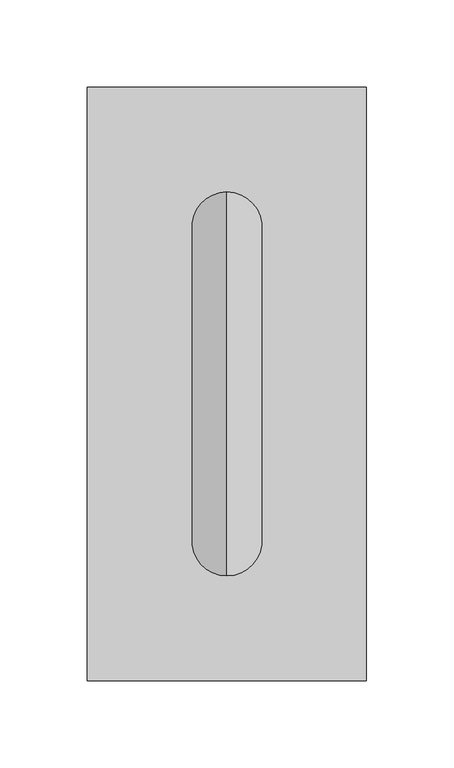
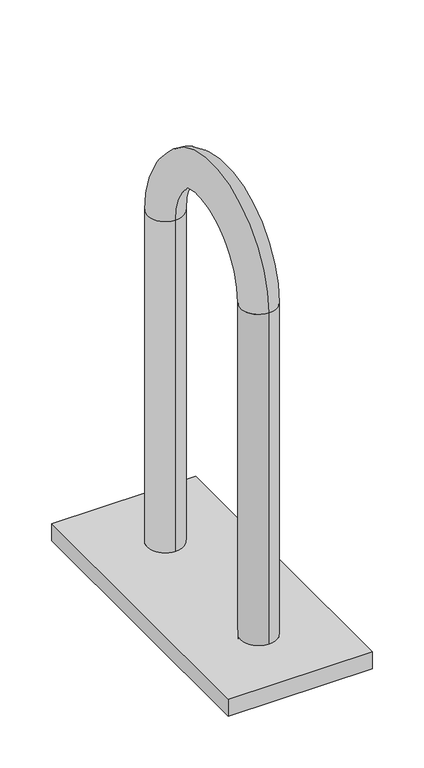
"""IFC4 building model written with IfcOpenShell, lengths in millimetres: proxy geometry, Опорный поручень : Опорный поручень для раковины."""

from ifc_helpers import new_model, si_unit, point, frame, origin, origin_with_axes, place, context, project, spatial, polyline, circle_curve, ellipse_curve, trimmed, outline, extrude, source, transform, mapped, element, save
from ifc_brep_helpers import plane_surface, cylinder_surface, revolved_surface, advanced_brep


def mechanical_equipment_83d53407(model_context):
    return source(origin(), model_context, "Body", "SolidModel", [
        extrude(outline(polyline([(80.0, 170.0), (80.0, -170.0), (-80.0, -170.0), (-80.0, 170.0), (80.0, 170.0)])), origin_with_axes(), (0.0, 0.0, 1.0), 20.0),
        advanced_brep(
        [(0.0, 110.0, 0.0), (0.0, 70.0, 0.0), (0.0, 110.0, 410.0), (0.0, 70.0, 410.0), (0.0, -70.0, 410.0), (0.0, -110.0, 410.0), (0.0, -110.0, 0.0), (0.0, -70.0, 0.0)],
        [
            (0, 1, circle_curve(frame((0.0, 90.0, 0.0), z_axis=(0.0, 0.0, -1.0), x_axis=(0.0, -1.0, 0.0)), 20.0)),
            (1, 0, circle_curve(frame((0.0, 90.0, 0.0), z_axis=(0.0, 0.0, -1.0), x_axis=(0.0, -1.0, 0.0)), 20.0)),
            (0, 2),
            (2, 3, circle_curve(frame((0.0, 90.0, 410.0), z_axis=(0.0, 0.0, -1.0), x_axis=(0.0, -1.0, 0.0)), 20.0)),
            (3, 1),
            (3, 2, circle_curve(frame((0.0, 90.0, 410.0), z_axis=(0.0, 0.0, -1.0), x_axis=(0.0, -1.0, 0.0)), 20.0)),
            (4, 3, circle_curve(frame((0.0, 0.0, 410.0), z_axis=(-1.0, 0.0, 0.0), x_axis=(0.0, 1.0, 0.0)), 70.0)),
            (2, 5, circle_curve(frame((0.0, 0.0, 410.0), z_axis=(1.0, 0.0, 0.0), x_axis=(0.0, 1.0, 0.0)), 110.0)),
            (5, 4, circle_curve(frame((0.0, -90.0, 410.0), z_axis=(0.0, 0.0, 1.0), x_axis=(0.0, 1.0, 0.0)), 20.0)),
            (4, 5, circle_curve(frame((0.0, -90.0, 410.0), z_axis=(0.0, 0.0, 1.0), x_axis=(0.0, 1.0, 0.0)), 20.0)),
            (6, 7, circle_curve(frame((0.0, -90.0, 0.0), z_axis=(0.0, 0.0, -1.0), x_axis=(0.0, 1.0, 0.0)), 20.0)),
            (7, 6, circle_curve(frame((0.0, -90.0, 0.0), z_axis=(0.0, 0.0, -1.0), x_axis=(0.0, 1.0, 0.0)), 20.0)),
            (5, 6),
            (7, 4),
        ],
        [
            plane_surface(frame((0.0, 90.0, 0.0), z_axis=(0.0, 0.0, -1.0), x_axis=(1.0, 0.0, 0.0))),
            cylinder_surface(frame((0.0, 90.0, 0.0), z_axis=(0.0, 0.0, -1.0), x_axis=(0.0, -1.0, 0.0)), 20.0),
            revolved_surface(trimmed(ellipse_curve(frame((0.0, 90.0, 410.0), z_axis=(0.0, 0.0, -1.0), x_axis=(0.0, -1.0, 0.0)), 20.0, 20.0), [point((0.0, 110.0, 410.0))], [point((0.0, 70.0, 410.0))], True, "CARTESIAN"), (0.0, 0.0, 410.0), (1.0, 0.0, 0.0)),
            revolved_surface(trimmed(ellipse_curve(frame((0.0, 90.0, 410.0), z_axis=(0.0, 0.0, -1.0), x_axis=(0.0, -1.0, 0.0)), 20.0, 20.0), [point((0.0, 70.0, 410.0))], [point((0.0, 110.0, 410.0))], True, "CARTESIAN"), (0.0, 0.0, 410.0), (1.0, 0.0, 0.0)),
            plane_surface(frame((0.0, -90.0, 0.0), z_axis=(0.0, 0.0, -1.0), x_axis=(1.0, 0.0, 0.0))),
            cylinder_surface(frame((0.0, -90.0, 410.0), z_axis=(0.0, 0.0, 1.0), x_axis=(0.0, 1.0, 0.0)), 20.0),
        ],
        [
            (0, [[1, 2]]),
            (1, [[-1, 3, 4, 5]]),
            (1, [[-2, -5, 6, -3]]),
            (2, [[7, -4, 8, 9]]),
            (3, [[-8, -6, -7, 10]]),
            (4, [[11, 12]]),
            (5, [[-9, 13, -12, 14]]),
            (5, [[-10, -14, -11, -13]]),
        ],
    ),
    ])


if __name__ == "__main__":
    model = new_model("IFC4")
    model_context = context("Model", 3, world=origin())
    ifc_project = project(units=[si_unit("LENGTHUNIT", "METRE", prefix="MILLI")], contexts=[model_context])
    site = spatial("IfcSite", under=ifc_project)
    building = spatial("IfcBuilding", under=site)
    placement = place(None, origin())
    mechanical_equipment_shape = mechanical_equipment_83d53407(model_context)
    element("IfcBuildingElementProxy", 1, Name="Опорный поручень : Опорный поручень для раковины", ObjectType="Опорный поручень : Опорный поручень для раковины", at=placement, inside=building, context=model_context, shape_type="MappedRepresentation", body=[
        mapped(mechanical_equipment_shape, transform((0.0, 0.0, 0.0), x_axis=(1.0, 0.0, 0.0), y_axis=(0.0, 1.0, 0.0), z_axis=(0.0, 0.0, 1.0))),
    ])
    save(model, "model.ifc")

# Revit data of these elements
# Type "Опорный поручень : Опорный поручень для раковины"
#   Model = "МГН"
#   Default Elevation = 1219.2 mm
#   ADSK_Размер_Длина = 500 mm
#   ADSK_Размер_Диаметр = 40 mm
#   ADSK_Размер_Высота = 180 mm
#   Откидной = no
#   ADSK_Материал = Сталь, нержавеющая, полированная
# Element 1 (IfcBuildingElementProxy, "Опорный поручень : Опорный поручень для раковины")
#   Materials on its faces: "Сталь, нержавеющая, полированная"
# Materials
#   "Сталь, нержавеющая, полированная": class "Металл", colour RGB 120 120 120, transparency 0, Description = "Сталь нержавеющая 18/8, полированная", Cost = 0
